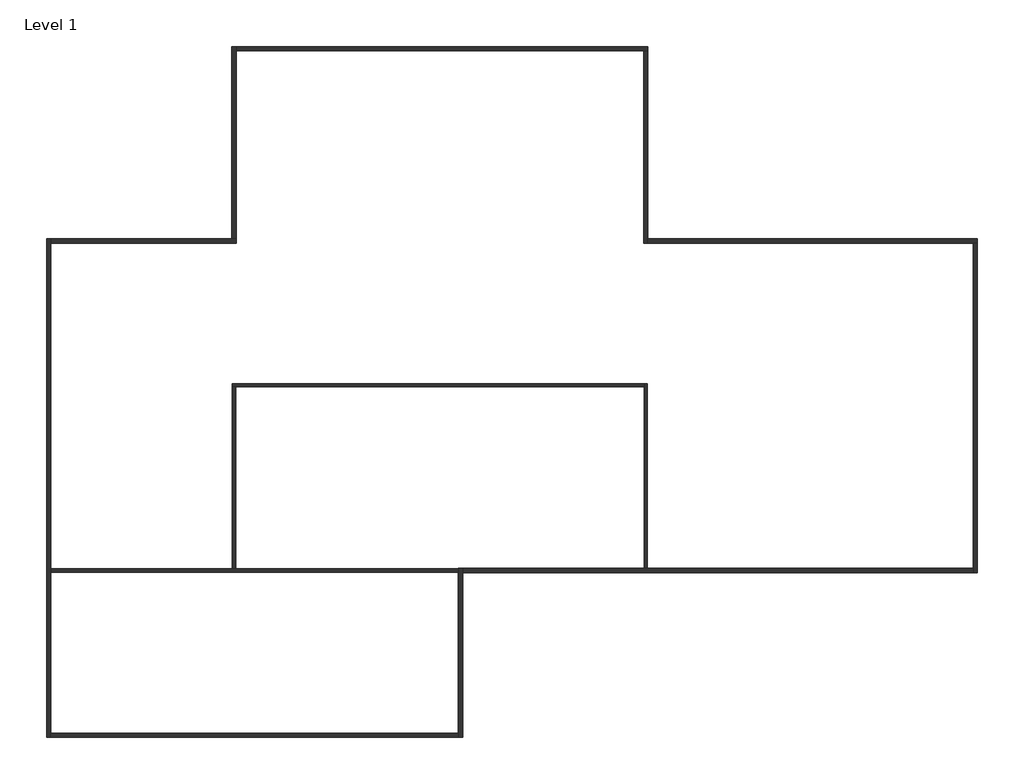
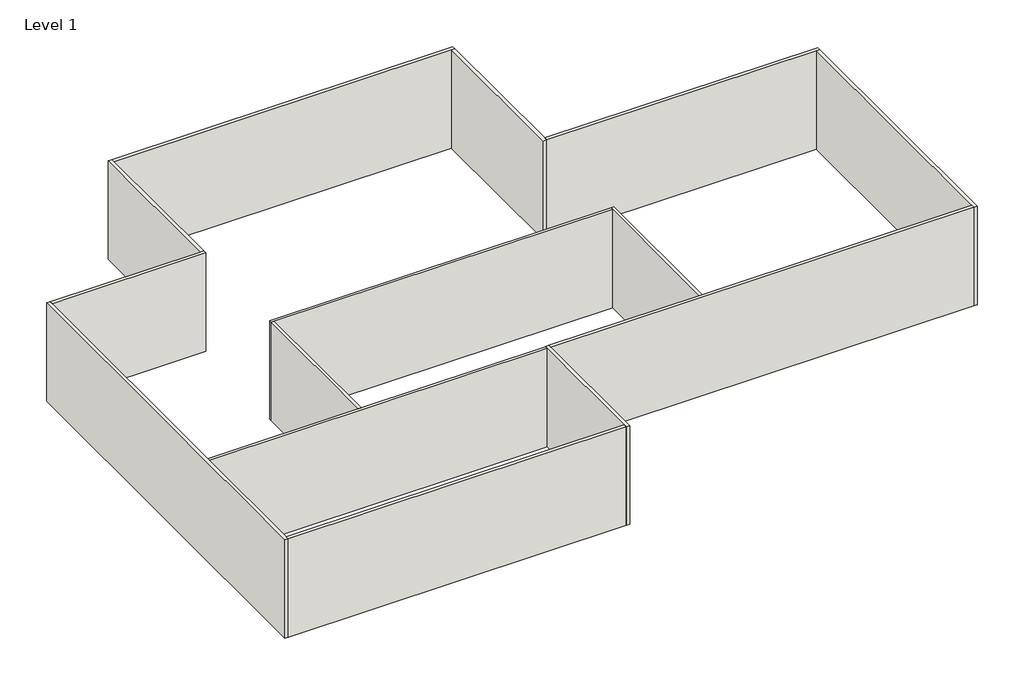
# One storey: 14 walls.
"""IFC4 building model written with IfcOpenShell, lengths in millimetres."""

from ifc_helpers import new_model, si_unit, origin, origin_with_axes, place, context, project, spatial, polyline, outline, extrude, faceted_brep, element, save

model = new_model("IFC4")

# Units and contexts
model_context = context("Model", 3, world=origin())
ifc_project = project(units=[si_unit("LENGTHUNIT", "METRE", prefix="MILLI")], contexts=[model_context])

# Site, building, storey
site = spatial("IfcSite", under=ifc_project)
building = spatial("IfcBuilding", under=site)
storey = spatial("IfcBuildingStorey", under=building, Name="Level 1", Elevation=0.0)

# Walls
placement = place(None, origin())
element("IfcWall", 1, ObjectType="Generic - 6\"", at=placement, inside=storey, context=model_context, shape_type="Brep", body=[
    faceted_brep([(6224.5657117, -9986.2030035, 0.0), (6224.5657117, -1011.6030035, 0.0), (6224.5657117, -1011.6030035, 6096.0), (6224.5657117, -9986.2030035, 6096.0), (6072.1657117, -9986.2030035, 0.0), (6072.1657117, -9986.2030035, 6096.0), (6072.1657117, -1164.0030035, 6096.0), (6072.1657117, -1011.6030035, 6096.0), (6072.1657117, -1011.6030035, 0.0), (6072.1657117, -1164.0030035, 0.0)], [[[0, 1, 2, 3]], [[4, 5, 6, 7, 8, 9]], [[1, 0, 4, 9, 8]], [[3, 2, 7, 6, 5]], [[0, 3, 5, 4]], [[2, 1, 8, 7]]]),
])
element("IfcWall", 2, ObjectType="Generic - 6\"", at=placement, inside=storey, context=model_context, shape_type="Brep", body=[
    faceted_brep([(6072.1657117, -1011.6030035, 0.0), (-13927.8342883, -1011.6030035, 0.0), (-13927.8342883, -1011.6030035, 6096.0), (6072.1657117, -1011.6030035, 6096.0), (6072.1657117, -1164.0030035, 0.0), (6072.1657117, -1164.0030035, 6096.0), (-13775.4342883, -1164.0030035, 6096.0), (-13927.8342883, -1164.0030035, 6096.0), (-13927.8342883, -1164.0030035, 0.0), (-13775.4342883, -1164.0030035, 0.0)], [[[0, 1, 2, 3]], [[4, 5, 6, 7, 8, 9]], [[1, 0, 4, 9, 8]], [[3, 2, 7, 6, 5]], [[0, 3, 5, 4]], [[2, 1, 8, 7]]]),
])
element("IfcWall", 3, ObjectType="Generic - 6\"", at=placement, inside=storey, context=model_context, shape_type="SweptSolid", body=[
    extrude(outline(polyline([(-13927.8342883, -10011.6030035), (-13927.8342883, -1164.0030035), (-13775.4342883, -1164.0030035), (-13775.4342883, -10011.6030035), (-13927.8342883, -10011.6030035)])), origin_with_axes(), (0.0, 0.0, 1.0), 6096.0),
])
element("IfcWall", 4, ObjectType="Generic - 6\"", at=placement, inside=storey, context=model_context, shape_type="Brep", body=[
    faceted_brep([(-2953.2342883, -10011.6030035, 0.0), (-13775.4342883, -10011.6030035, 0.0), (-13927.8342883, -10011.6030035, 0.0), (-22750.0342883, -10011.6030035, 0.0), (-22750.0342883, -10011.6030035, 6096.0), (-13927.8342883, -10011.6030035, 6096.0), (-13775.4342883, -10011.6030035, 6096.0), (-2953.2342883, -10011.6030035, 6096.0), (-2953.2342883, -10164.0030035, 0.0), (-2953.2342883, -10164.0030035, 6096.0), (-22750.0342883, -10164.0030035, 6096.0), (-22750.0342883, -10164.0030035, 0.0)], [[[0, 1, 2, 3, 4, 5, 6, 7]], [[8, 9, 10, 11]], [[3, 2, 1, 0, 8, 11]], [[7, 6, 5, 4, 10, 9]], [[4, 3, 11, 10]], [[0, 7, 9, 8]]]),
])
element("IfcWall", 5, ObjectType="Generic - 8\"", at=placement, inside=storey, context=model_context, shape_type="Brep", body=[
    faceted_brep([(-22750.0342883, -18189.4030035, 0.0), (-22750.0342883, -17986.2030035, 0.0), (-22750.0342883, -10164.0030035, 0.0), (-22750.0342883, -10011.6030035, 0.0), (-22750.0342883, 5810.5969965, 0.0), (-22750.0342883, 6013.7969965, 0.0), (-22750.0342883, 6013.7969965, 6096.0), (-22750.0342883, 5810.5969965, 6096.0), (-22750.0342883, -10011.6030035, 6096.0), (-22750.0342883, -10164.0030035, 6096.0), (-22750.0342883, -17986.2030035, 6096.0), (-22750.0342883, -18189.4030035, 6096.0), (-22953.2342883, -18189.4030035, 0.0), (-22953.2342883, -18189.4030035, 6096.0), (-22953.2342883, 6013.7969965, 6096.0), (-22953.2342883, 6013.7969965, 0.0)], [[[0, 1, 2, 3, 4, 5, 6, 7, 8, 9, 10, 11]], [[12, 13, 14, 15]], [[5, 4, 3, 2, 1, 0, 12, 15]], [[11, 10, 9, 8, 7, 6, 14, 13]], [[6, 5, 15, 14]], [[0, 11, 13, 12]]]),
])
element("IfcWall", 6, ObjectType="Generic - 8\"", at=placement, inside=storey, context=model_context, shape_type="Brep", body=[
    faceted_brep([(-22750.0342883, 5810.5969965, 0.0), (-13750.0342883, 5810.5969965, 0.0), (-13750.0342883, 5810.5969965, 6096.0), (-22750.0342883, 5810.5969965, 6096.0), (-22750.0342883, 6013.7969965, 0.0), (-22750.0342883, 6013.7969965, 6096.0), (-13953.2342883, 6013.7969965, 6096.0), (-13750.0342883, 6013.7969965, 6096.0), (-13750.0342883, 6013.7969965, 0.0), (-13953.2342883, 6013.7969965, 0.0)], [[[0, 1, 2, 3]], [[4, 5, 6, 7, 8, 9]], [[1, 0, 4, 9, 8]], [[3, 2, 7, 6, 5]], [[0, 3, 5, 4]], [[2, 1, 8, 7]]]),
])
element("IfcWall", 7, ObjectType="Generic - 8\"", at=placement, inside=storey, context=model_context, shape_type="Brep", body=[
    faceted_brep([(-13750.0342883, 6013.7969965, 0.0), (-13750.0342883, 15150.4244043, 0.0), (-13750.0342883, 15353.6244043, 0.0), (-13750.0342883, 15353.6244043, 6096.0), (-13750.0342883, 15150.4244043, 6096.0), (-13750.0342883, 6013.7969965, 6096.0), (-13953.2342883, 6013.7969965, 0.0), (-13953.2342883, 6013.7969965, 6096.0), (-13953.2342883, 15353.6244043, 6096.0), (-13953.2342883, 15353.6244043, 0.0)], [[[0, 1, 2, 3, 4, 5]], [[6, 7, 8, 9]], [[2, 1, 0, 6, 9]], [[5, 4, 3, 8, 7]], [[0, 5, 7, 6]], [[3, 2, 9, 8]]]),
])
element("IfcWall", 8, ObjectType="Generic - 8\"", at=placement, inside=storey, context=model_context, shape_type="Brep", body=[
    faceted_brep([(-13750.0342883, 15150.4244043, 0.0), (6046.7657117, 15150.4244043, 0.0), (6249.9657117, 15150.4244043, 0.0), (6249.9657117, 15150.4244043, 6096.0), (6046.7657117, 15150.4244043, 6096.0), (-13750.0342883, 15150.4244043, 6096.0), (-13750.0342883, 15353.6244043, 0.0), (-13750.0342883, 15353.6244043, 6096.0), (6249.9657117, 15353.6244043, 6096.0), (6249.9657117, 15353.6244043, 0.0)], [[[0, 1, 2, 3, 4, 5]], [[6, 7, 8, 9]], [[2, 1, 0, 6, 9]], [[5, 4, 3, 8, 7]], [[0, 5, 7, 6]], [[3, 2, 9, 8]]]),
])
element("IfcWall", 9, ObjectType="Generic - 8\"", at=placement, inside=storey, context=model_context, shape_type="Brep", body=[
    faceted_brep([(6046.7657117, 15150.4244043, 0.0), (6046.7657117, 5810.5969965, 0.0), (6046.7657117, 5810.5969965, 6096.0), (6046.7657117, 15150.4244043, 6096.0), (6249.9657117, 15150.4244043, 0.0), (6249.9657117, 15150.4244043, 6096.0), (6249.9657117, 6013.7969965, 6096.0), (6249.9657117, 5810.5969965, 6096.0), (6249.9657117, 5810.5969965, 0.0), (6249.9657117, 6013.7969965, 0.0)], [[[0, 1, 2, 3]], [[4, 5, 6, 7, 8, 9]], [[1, 0, 4, 9, 8]], [[3, 2, 7, 6, 5]], [[0, 3, 5, 4]], [[2, 1, 8, 7]]]),
])
element("IfcWall", 10, ObjectType="Generic - 8\"", at=placement, inside=storey, context=model_context, shape_type="Brep", body=[
    faceted_brep([(6249.9657117, 5810.5969965, 0.0), (22046.7657117, 5810.5969965, 0.0), (22249.9657117, 5810.5969965, 0.0), (22249.9657117, 5810.5969965, 6096.0), (22046.7657117, 5810.5969965, 6096.0), (6249.9657117, 5810.5969965, 6096.0), (6249.9657117, 6013.7969965, 0.0), (6249.9657117, 6013.7969965, 6096.0), (22249.9657117, 6013.7969965, 6096.0), (22249.9657117, 6013.7969965, 0.0)], [[[0, 1, 2, 3, 4, 5]], [[6, 7, 8, 9]], [[2, 1, 0, 6, 9]], [[5, 4, 3, 8, 7]], [[0, 5, 7, 6]], [[3, 2, 9, 8]]]),
])
element("IfcWall", 11, ObjectType="Generic - 8\"", at=placement, inside=storey, context=model_context, shape_type="Brep", body=[
    faceted_brep([(22046.7657117, 5810.5969965, 0.0), (22046.7657117, -9986.2030035, 0.0), (22046.7657117, -10189.4030035, 0.0), (22046.7657117, -10189.4030035, 6096.0), (22046.7657117, -9986.2030035, 6096.0), (22046.7657117, 5810.5969965, 6096.0), (22249.9657117, 5810.5969965, 0.0), (22249.9657117, 5810.5969965, 6096.0), (22249.9657117, -10189.4030035, 6096.0), (22249.9657117, -10189.4030035, 0.0)], [[[0, 1, 2, 3, 4, 5]], [[6, 7, 8, 9]], [[2, 1, 0, 6, 9]], [[5, 4, 3, 8, 7]], [[0, 5, 7, 6]], [[3, 2, 9, 8]]]),
])
element("IfcWall", 12, ObjectType="Generic - 8\"", at=placement, inside=storey, context=model_context, shape_type="Brep", body=[
    faceted_brep([(22046.7657117, -9986.2030035, 0.0), (6224.5657117, -9986.2030035, 0.0), (6072.1657117, -9986.2030035, 0.0), (-2750.0342883, -9986.2030035, 0.0), (-2750.0342883, -9986.2030035, 6096.0), (6072.1657117, -9986.2030035, 6096.0), (6224.5657117, -9986.2030035, 6096.0), (22046.7657117, -9986.2030035, 6096.0), (22046.7657117, -10189.4030035, 0.0), (22046.7657117, -10189.4030035, 6096.0), (-2750.0342883, -10189.4030035, 6096.0), (-2750.0342883, -10189.4030035, 0.0)], [[[0, 1, 2, 3, 4, 5, 6, 7]], [[8, 9, 10, 11]], [[3, 2, 1, 0, 8, 11]], [[7, 6, 5, 4, 10, 9]], [[0, 7, 9, 8]], [[4, 3, 11, 10]]]),
])
element("IfcWall", 13, ObjectType="Generic - 8\"", at=placement, inside=storey, context=model_context, shape_type="Brep", body=[
    faceted_brep([(-2953.2342883, -9986.2030035, 0.0), (-2953.2342883, -10011.6030035, 0.0), (-2953.2342883, -10164.0030035, 0.0), (-2953.2342883, -17986.2030035, 0.0), (-2953.2342883, -18189.4030035, 0.0), (-2953.2342883, -18189.4030035, 6096.0), (-2953.2342883, -17986.2030035, 6096.0), (-2953.2342883, -10164.0030035, 6096.0), (-2953.2342883, -10011.6030035, 6096.0), (-2953.2342883, -9986.2030035, 6096.0), (-2750.0342883, -9986.2030035, 0.0), (-2750.0342883, -9986.2030035, 6096.0), (-2750.0342883, -10189.4030035, 6096.0), (-2750.0342883, -18189.4030035, 6096.0), (-2750.0342883, -18189.4030035, 0.0), (-2750.0342883, -10189.4030035, 0.0)], [[[0, 1, 2, 3, 4, 5, 6, 7, 8, 9]], [[10, 11, 12, 13, 14, 15]], [[4, 3, 2, 1, 0, 10, 15, 14]], [[9, 8, 7, 6, 5, 13, 12, 11]], [[5, 4, 14, 13]], [[0, 9, 11, 10]]]),
])
element("IfcWall", 14, ObjectType="Generic - 8\"", at=placement, inside=storey, context=model_context, shape_type="SweptSolid", body=[
    extrude(outline(polyline([(-22750.0342883, -17986.2030035), (-2953.2342883, -17986.2030035), (-2953.2342883, -18189.4030035), (-22750.0342883, -18189.4030035), (-22750.0342883, -17986.2030035)])), origin_with_axes(), (0.0, 0.0, 1.0), 6096.0),
])

save(model, "model.ifc")

# Revit data of these elements
# Project information
#   Project Issue Date = "Issue Date"
#   Project Status = "Project Status"
#   Client Name = "Owner"
#   Project Address = "Enter address here"
#   Project Name = "Project Name"
#   Project Number = "Project Number"
# Type "Generic - 6\""
#   Assembly Code = "B2010"
#   Layers, outside or top first: 0.1524 m no material (function 1)
# Type "Generic - 8\""
#   Assembly Code = "B2010"
#   Layers, outside or top first: 0.2032 m no material (function 1)
# Elements 1, 2, 3, 4 (IfcWall, "Generic - 6\"")
#   Top Offset = 0 m
#   Base Offset = 0 m
#   Unconnected Height = 6.096 m
#   wall height = 6.096 m
#   Phase Created = New Construction
#   Base Constraint = Level 1
#   Materials on its faces: "Default Wall"
# Elements 5, 6, 7, 8, 9, 10, 11, 12, 13, 14 (IfcWall, "Generic - 8\"")
#   Top Offset = 0 m
#   Base Offset = 0 m
#   Unconnected Height = 6.096 m
#   wall height = 6.096 m
#   Phase Created = New Construction
#   Base Constraint = Level 1
#   Materials on its faces: "Default Wall"
# Materials
#   "Default Wall": class "Miscellaneous", colour RGB 128 128 128, transparency 0, Cost = 0
